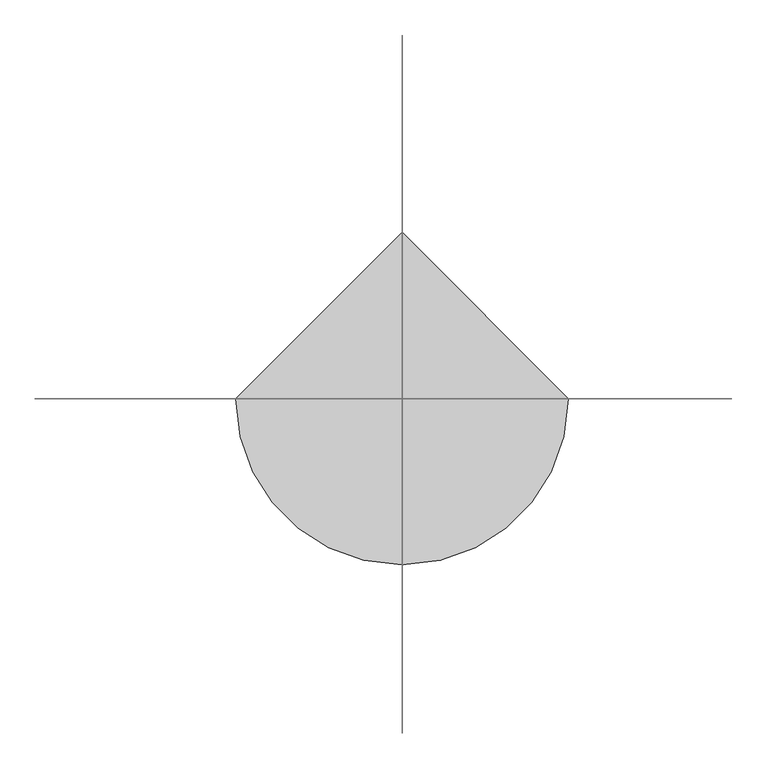
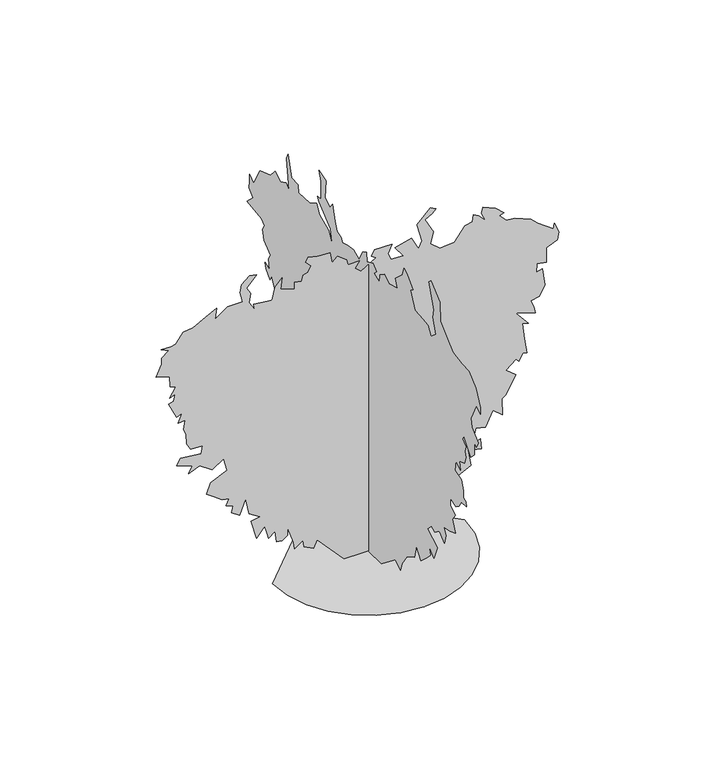
"""IFC4 building model written with IfcOpenShell, lengths in millimetres: proxy geometry, meadowlark 26084 : meadowlark 26084."""

import ifcopenshell
import ifcopenshell.guid

model = None  # the IFC model being written
_history = None  # IfcOwnerHistory: only IFC2X3 demands one
_inside = {}  # id of a spatial element -> (the spatial element, [elements in it])
_under = {}  # id of a project, library or spatial element -> (it, [spatial elements below it])
_declared = {}  # id of a project -> (the project, [libraries it declares])
_typed = {}  # id of a type object -> (the type object, [elements of that type])
_made_of = {}  # id of a material, layer set ... -> (it, [elements and type objects made of it])


def new_model(schema):
    """Start an empty IFC model of exactly this schema.

    Asked for "IFC4X3", IfcOpenShell would pick the latest addendum, in which some entities
    have other attributes; the version numbers below select the first issue.
    IFC2X3 requires an IfcOwnerHistory on every rooted entity: one is made here for all.
    """
    global model, _history
    if schema == "IFC4X3":
        model = ifcopenshell.file(schema_version=(4, 3, 0, 0))
    else:
        model = ifcopenshell.file(schema=schema)
    _inside.clear()
    _under.clear()
    _declared.clear()
    _typed.clear()
    _made_of.clear()
    _history = None
    if model.schema == "IFC2X3":
        org = make("IfcOrganization", Name="unknown")
        user = make(
            "IfcPersonAndOrganization",
            ThePerson=make("IfcPerson", FamilyName="unknown"),
            TheOrganization=org,
        )
        app = make(
            "IfcApplication",
            ApplicationDeveloper=org,
            Version="unknown",
            ApplicationFullName="unknown",
            ApplicationIdentifier="unknown",
        )
        _history = make(
            "IfcOwnerHistory",
            OwningUser=user,
            OwningApplication=app,
            ChangeAction="ADDED",
            CreationDate=0,
        )
    return model


def make(cls, **values):
    """One entity of the class cls with the attributes given. An attribute that is None is left unset."""
    return model.create_entity(
        cls, **{name: value for name, value in values.items() if value is not None}
    )


def rooted(cls, **values):
    """An entity with a GlobalId (a new one), such as an element, a storey or a relation."""
    return make(cls, GlobalId=ifcopenshell.guid.new(), OwnerHistory=_history, **values)


def si_unit(unit_type, name, prefix=None):
    """IfcSIUnit, for example si_unit("LENGTHUNIT", "METRE", prefix="MILLI")."""
    return make("IfcSIUnit", UnitType=unit_type, Prefix=prefix, Name=name)


def assignment(units):
    """IfcUnitAssignment: the units of a project."""
    return None if units is None else make("IfcUnitAssignment", Units=units)


def point(xyz):
    """IfcCartesianPoint."""
    return None if xyz is None else make("IfcCartesianPoint", Coordinates=xyz)


def direction(xyz):
    """IfcDirection."""
    return None if xyz is None else make("IfcDirection", DirectionRatios=xyz)


def frame(location, z_axis=None, x_axis=None):
    """IfcAxis2Placement3D, a coordinate frame: its origin and axes. An axis left out is left unset."""
    return make(
        "IfcAxis2Placement3D",
        Location=point(location),
        Axis=direction(z_axis),
        RefDirection=direction(x_axis),
    )


def origin():
    """The frame at (0, 0, 0) with its axes left unset."""
    return frame((0.0, 0.0, 0.0))


def place(relative_to, where):
    """IfcLocalPlacement: puts the frame where relative to a parent placement (None: the world)."""
    return make(
        "IfcLocalPlacement", PlacementRelTo=relative_to, RelativePlacement=where
    )


def context(
    kind, dimensions, precision=None, world=None, true_north=None, identifier=None
):
    """IfcGeometricRepresentationContext, for example the 3D "Model" context."""
    return make(
        "IfcGeometricRepresentationContext",
        ContextIdentifier=identifier,
        ContextType=kind,
        CoordinateSpaceDimension=dimensions,
        Precision=precision,
        WorldCoordinateSystem=world,
        TrueNorth=true_north,
    )


def project(units=None, contexts=None):
    """IfcProject with its units and contexts."""
    return rooted(
        "IfcProject",
        Name="project",
        RepresentationContexts=contexts,
        UnitsInContext=assignment(units),
    )


def spatial(cls, under=None, at=None, **own):
    """A site, building, storey or space (cls), placed at a placement, below another one or the project."""
    s = rooted(cls, ObjectPlacement=at, **own)
    if under is not None:
        _under.setdefault(under.id(), (under, []))[1].append(s)
    return s


def point_list(points):
    """IfcCartesianPointList2D or 3D."""
    cls = (
        "IfcCartesianPointList2D" if len(points[0]) == 2 else "IfcCartesianPointList3D"
    )
    return make(cls, CoordList=points)


def triangles(points, corners, closed=None, point_numbers=None):
    """IfcTriangulatedFaceSet: each triangle names its three corners, points numbered from 1."""
    return make(
        "IfcTriangulatedFaceSet",
        Coordinates=point_list(points),
        Closed=closed,
        CoordIndex=corners,
        PnIndex=point_numbers,
    )


def shape(context_of_items, identifier, shape_type, items):
    """IfcShapeRepresentation: the items that make up one representation, for example the "Body"."""
    return make(
        "IfcShapeRepresentation",
        ContextOfItems=context_of_items,
        RepresentationIdentifier=identifier,
        RepresentationType=shape_type,
        Items=items,
    )


def source(mapping_origin, context_of_items, identifier, shape_type, items):
    """IfcRepresentationMap: a shape defined once, which mapped items show again and again."""
    return make(
        "IfcRepresentationMap",
        MappingOrigin=mapping_origin,
        MappedRepresentation=shape(context_of_items, identifier, shape_type, items),
    )


def transform(
    local_origin,
    x_axis=None,
    y_axis=None,
    z_axis=None,
    scale=None,
    scale2=None,
    scale3=None,
    uniform=True,
):
    """IfcCartesianTransformationOperator3D, or its non-uniform kind. x_axis, y_axis, z_axis: its Axis1, 2, 3."""
    if uniform:
        return make(
            "IfcCartesianTransformationOperator3D",
            Axis1=direction(x_axis),
            Axis2=direction(y_axis),
            LocalOrigin=point(local_origin),
            Scale=scale,
            Axis3=direction(z_axis),
        )
    return make(
        "IfcCartesianTransformationOperator3DnonUniform",
        Axis1=direction(x_axis),
        Axis2=direction(y_axis),
        LocalOrigin=point(local_origin),
        Scale=scale,
        Axis3=direction(z_axis),
        Scale2=scale2,
        Scale3=scale3,
    )


def mapped(mapping_source, mapping_target):
    """IfcMappedItem: shows the shape of a source again, moved by a transform."""
    return make(
        "IfcMappedItem", MappingSource=mapping_source, MappingTarget=mapping_target
    )


def made_of(thing, what):
    """Note that an element or type object is made of a material, layer set ...; save() writes the relation."""
    if what is not None:
        _made_of.setdefault(what.id(), (what, []))[1].append(thing)
    return thing


def element(
    cls,
    number,
    at=None,
    inside=None,
    cuts=None,
    type_object=None,
    material=None,
    context=None,
    identifier="Body",
    shape_type=None,
    held_by="IfcProductDefinitionShape",
    body=None,
    shapes=None,
    **own,
):
    """One element of the class cls, such as IfcWall. Its Tag is "e" and its number.

    at: its placement. inside: the storey or other place that contains it. cuts: it is an
    opening in that element (IfcRelVoidsElement). A single representation is given by context,
    identifier, shape_type and body (its items); several are given by shapes. held_by: the class
    of the entity that holds the representations. save() writes the other relations.
    """
    e = rooted(cls, Tag="e%d" % number, ObjectPlacement=at, **own)
    if body is not None:
        shapes = [shape(context, identifier, shape_type, body)]
    if shapes is not None:
        e.Representation = make(held_by, Representations=shapes)
    if inside is not None:
        _inside.setdefault(inside.id(), (inside, []))[1].append(e)
    if cuts is not None:
        rooted(
            "IfcRelVoidsElement", RelatingBuildingElement=cuts, RelatedOpeningElement=e
        )
    if type_object is not None:
        _typed.setdefault(type_object.id(), (type_object, []))[1].append(e)
    return made_of(e, material)


def aggregate(whole, parts):
    """IfcRelAggregates: a whole, such as a stair, and the parts it consists of."""
    return rooted("IfcRelAggregates", RelatingObject=whole, RelatedObjects=parts)


def save(model, path):
    """Write the relations noted so far, then the file.

    IfcRelAggregates (storeys below a building ...), IfcRelContainedInSpatialStructure (elements
    in a storey), IfcRelDefinesByType, IfcRelAssociatesMaterial and IfcRelDeclares: one each for
    every whole, place, type object, material and project.
    """
    for whole, parts in _under.values():
        aggregate(whole, parts)
    for where, things in _inside.values():
        rooted(
            "IfcRelContainedInSpatialStructure",
            RelatedElements=things,
            RelatingStructure=where,
        )
    for kind, things in _typed.values():
        rooted("IfcRelDefinesByType", RelatedObjects=things, RelatingType=kind)
    for what, things in _made_of.values():
        rooted("IfcRelAssociatesMaterial", RelatedObjects=things, RelatingMaterial=what)
    for by, libraries in _declared.values():
        rooted("IfcRelDeclares", RelatingContext=by, RelatedDefinitions=libraries)
    model.write(path)


def entourage_9ef344a8(model_context):
    return source(origin(), model_context, "Body", "Tessellation", [
        triangles([(-63.9369313, 2.6e-06, 2.5813025), (-98.6351404, 1.9e-06, 41.3616468), (-133.3335948, 1.1e-06, 80.1421467), (-143.538813, 2.7e-06, 59.7314513), (-168.0315495, 3.1e-06, 71.9778149), (-170.0726858, 2.1e-06, 90.347365), (-192.5245312, 3.9e-06, 76.0598514), (-194.5656857, 2.9e-06, 94.4296558), (-210.8940858, 9e-07, 139.3333375), (-210.8940858, 2.1e-06, 118.9223832), (-225.1818402, 3.4e-06, 108.7171649), (-239.469104, 3.9e-06, 110.7583103), (-243.5513948, 2.2e-06, 141.3742286), (-260.2917792, 3.7e-06, 128.4682213), (-264.2033864, 3e-06, 143.1357217), (-270.0860397, 2e-06, 163.8260649), (-290.4949502, 4.4e-06, 139.3333375), (-304.7824684, 2e-06, 190.3599468), (-282.331386, 8e-07, 194.4422376), (-310.9064223, 9e-07, 212.8117922), (-319.0699865, -1.4e-06, 257.7162279), (-335.3996584, 1.7e-06, 216.894083), (-355.8110942, 1.8e-06, 231.181583), (-351.7293303, 5e-07, 249.5511376), (-370.0986305, 9e-07, 255.674056), (-361.9325229, -4e-07, 272.003746), (-380.3043303, 2e-07, 276.0855281), (-401.9400736, 2e-07, 291.703997), (-421.1247311, 3e-07, 304.6605463), (-410.918995, -1.9e-06, 333.2355826), (-368.1987102, -4.9e-06, 351.9401459), (-376.2200229, -6.6e-06, 386.3038187), (-406.8371947, -4.1e-06, 367.9345184), (-439.493995, -4.1e-06, 390.385619), (-468.0690313, -2.1e-06, 378.137711), (-457.8632953, -3.5e-06, 394.4673829), (-498.6862032, -2.7e-06, 410.7970548), (-488.4805035, -4.1e-06, 427.1242195), (-435.4122311, -6.1e-06, 421.0002474), (-431.3304308, -7.5e-06, 441.4117195), (-461.9450955, -6.2e-06, 443.4538914), (-472.1508316, -6.9e-06, 461.8231553), (-474.1929671, -8.4e-06, 488.3560198), (-480.3169393, -9e-06, 502.6435561), (-476.2325955, -1.06e-05, 527.1367922), (-495.4832737, -9.7e-06, 526.35192), (-484.3987032, -1.16e-05, 549.5878564), (-498.6862032, -1.06e-05, 543.466464), (-519.0951319, -1.23e-05, 586.3290004), (-506.8497674, -1.3e-05, 590.4107643), (-502.7680035, -1.43e-05, 608.7800646), (-517.0555035, -1.33e-05, 602.6561288), (-500.7258316, -1.55e-05, 627.1493649), (-516.1995237, -1.52e-05, 634.2689884), (-517.0555035, -1.68e-05, 661.848337), (-551.7544756, -1.59e-05, 672.0540367), (-537.4644321, -1.84e-05, 702.6687378), (-538.1857907, -1.94e-05, 720.3319038), (-519.0951319, -2.1e-05, 733.2859097), (-539.506604, -2.07e-05, 743.4916094), (-512.7375257, -2.18e-05, 742.0895147), (-500.7258316, -2.25e-05, 745.5312378), (-482.3565313, -2.49e-05, 772.0666094), (-455.8236669, -2.62e-05, 774.1062378), (-423.1668666, -2.87e-05, 792.4755381), (-395.1176339, -3.08e-05, 806.3871162), (-398.6736305, -2.9e-05, 778.1880381), (-366.0168303, -3.17e-05, 800.6416821), (-327.2360942, -3.34e-05, 800.6416821), (-334.4166515, -3.47e-05, 827.9339842), (-330.1088113, -3.62e-05, 849.0616917), (-308.8667939, -3.81e-05, 865.9552826), (-290.4949502, -3.87e-05, 861.8734823), (-317.5358142, -3.58e-05, 834.0731443), (-306.8246221, -3.53e-05, 816.9688105), (-310.9064223, -3.36e-05, 792.4755381), (-296.6189042, -3.29e-05, 770.0245102), (-298.6610579, -3.37e-05, 784.3120102), (-251.0357672, -3.54e-05, 778.383593), (-243.5513948, -3.77e-05, 810.8473818), (-225.1818402, -3.97e-05, 831.2563105), (-228.2958943, -3.78e-05, 801.312208), (-192.5245312, -3.86e-05, 788.3937378), (-192.5245312, -3.97e-05, 806.7630381), (-173.5245645, -4.03e-05, 803.1613684), (-170.0726858, -4.14e-05, 819.0109823), (-157.8260678, -4.22e-05, 823.0927099), (-149.662004, -4.34e-05, 837.3802826), (-163.9495131, -4.36e-05, 851.6677826), (-157.8260678, -4.46e-05, 863.9131107), (-131.292195, -4.54e-05, 857.7916821), (-100.6760314, -4.66e-05, 855.7495102), (-94.5528496, -4.52e-05, 827.1745102), (-80.2653314, -4.65e-05, 839.4223818), (-56.9158573, -4.65e-05, 821.1673914), (-53.7314587, -4.57e-05, 806.7630381), (-23.1153655, -4.71e-05, 806.7630381), (-35.3616542, -4.56e-05, 790.4359097), (-19.0331746, -4.54e-05, 776.1484097), (19.7470164, -4.86e-05, 800.6416821), (7.5007532, -4.85e-05, 808.8052099), (15.1231208, -4.98e-05, 823.890263), (60.5683824, -5.17e-05, 823.0927099), (50.5958261, -4.99e-05, 799.816151), (58.5274868, -4.92e-05, 782.2723818), (91.1845505, -5.05e-05, 780.2302099), (68.732964, -5.13e-05, 810.8473818), (111.5952414, -5.38e-05, 821.0506107), (129.9650504, -5.25e-05, 786.3541821), (138.9452253, -5.4e-05, 804.6625122), (125.8830048, -5.64e-05, 853.7099545), (160.581223, -6e-05, 888.4063831), (174.868723, -6.01e-05, 880.2427826), (164.6635138, -5.91e-05, 870.0370829), (146.2937048, -5.76e-05, 859.8313105), (168.7455503, -5.62e-05, 819.0109823), (161.0930195, -5.4e-05, 788.6985884), (185.0742047, -5.39e-05, 767.9848818), (203.4434868, -5.48e-05, 770.0245102), (223.8544503, -5.58e-05, 772.0666094), (250.3885683, -5.9e-05, 806.7630381), (269.7101179, -6.01e-05, 811.2766434), (272.8393963, -6.13e-05, 829.2166821), (285.0872861, -6.15e-05, 823.0927099), (304.0839645, -6.12e-05, 803.1613684), (293.2508503, -6.21e-05, 827.1745102), (297.3326324, -6.31e-05, 841.4620102), (329.9894508, -6.37e-05, 827.1745102), (351.394031, -6.35e-05, 807.9441433), (340.0529354, -6.27e-05, 803.4457987), (358.5644508, -6.24e-05, 784.3120102), (381.0180948, -6.33e-05, 782.2723818), (422.1051581, -6.41e-05, 765.7470823), (440.2077596, -6.38e-05, 747.5734097), (481.0306675, -6.39e-05, 718.9984097), (483.0702959, -6.48e-05, 733.2859097), (495.3181675, -6.36e-05, 704.710837), (491.2364036, -6.23e-05, 684.2994375), (462.6588238, -6.03e-05, 672.0540367), (462.6588238, -5.8e-05, 633.273337), (438.1681312, -5.71e-05, 637.3550646), (436.1259593, -5.57e-05, 614.9040367), (452.4556312, -5.67e-05, 618.9857643), (458.5770598, -5.41e-05, 572.041464), (444.2895235, -5.19e-05, 545.5060925), (421.8384593, -5.07e-05, 541.4242922), (430.0020235, -4.98e-05, 521.0128201), (434.0863309, -4.91e-05, 504.6856916), (383.0577232, -4.78e-05, 521.0128201), (415.7145235, -4.69e-05, 482.2346274), (399.3873951, -4.64e-05, 486.3163914), (405.5087874, -4.42e-05, 443.4538914), (411.6327232, -4.2e-05, 402.6309471), (401.4269872, -4.17e-05, 404.673119), (391.2212874, -4.01e-05, 386.3038187), (383.0577232, -4.03e-05, 394.4673829), (356.5248588, -3.79e-05, 374.0559471), (383.0577232, -3.77e-05, 351.6048466), (356.5248588, -3.39e-05, 306.7001747), (346.3191227, -3.29e-05, 298.5365923), (348.3587511, -3.03e-05, 253.6334284), (323.4463909, -3.05e-05, 274.9933165), (303.4565864, -2.73e-05, 235.2636194), (278.9633503, -2.66e-05, 241.3868104), (266.8272088, -2.35e-05, 199.2829668), (291.2086966, -2.52e-05, 208.7297557), (293.2508503, -2.36e-05, 180.1547194), (258.5518782, -2.25e-05, 188.3190466), (266.7179858, -2.02e-05, 143.415374), (232.0187775, -1.77e-05, 127.0867195), (215.6903774, -1.54e-05, 100.5528377), (197.3205684, -1.5e-05, 106.6760195), (191.1973775, -1.2e-05, 61.7723423), (176.9098775, -1.3e-05, 88.306474), (150.3759956, -8.8e-06, 37.2796104), (132.0059414, -8.8e-06, 51.5671195), (68.732964, -3.2e-06, 2.5813025), (5e-07, 58.5086925, 0.0), (5.6e-06, 119.7410287, 55.1089), (6.1e-06, 137.5863239, 49.658565), (5.6e-06, 170.7679014, 104.0948725), (5.5e-06, 180.9731106, 91.8482545), (9.8e-06, 197.3017651, 73.4787044), (6.8e-06, 213.6304195, 87.7662181), (6.7e-06, 205.4660923, 93.8893999), (9.7e-06, 223.8356469, 144.9162635), (8.6e-06, 231.9999742, 112.2589454), (1e-05, 238.1231651, 136.7519272), (1.13e-05, 276.9033925, 128.5875999), (1.12e-05, 254.4523283, 148.9982999), (1.22e-05, 274.8637822, 151.0394453), (1.45e-05, 307.5205825, 171.4501453), (1.42e-05, 280.9851927, 191.8608363), (1.68e-05, 299.3544748, 232.6824725), (1.68e-05, 317.7263186, 214.3126635), (1.89e-05, 350.3043809, 228.0708535), (1.99e-05, 340.1773828, 261.2569819), (2.07e-05, 354.4649191, 265.338764), (2.22e-05, 356.5045112, 297.9955825), (2.36e-05, 393.2456552, 293.9138004), (2.61e-05, 411.6149554, 332.6945546), (2.58e-05, 397.3274554, 338.8184904), (2.92e-05, 438.1478199, 377.5992265), (2.82e-05, 405.4910196, 385.7627907), (2.9e-05, 411.6149554, 398.0081552), (2.55e-05, 417.7363478, 412.2956552), (2.48e-05, 395.2852836, 418.4196273), (2.73e-05, 415.6967194, 455.1581915), (2.98e-05, 436.1081915, 491.8993355), (2.95e-05, 444.2717557, 477.6118355), (3.11e-05, 460.5988841, 498.0207278), (3.2e-05, 466.7228199, 512.3082642), (3.07e-05, 446.3113841, 504.1447), (3.21e-05, 450.3956915, 530.6800715), (3.24e-05, 440.1899554, 547.0072), (3.47e-05, 470.8046202, 569.4583005), (3.61e-05, 476.928556, 595.9937084), (3.64e-05, 468.7649918, 610.2812084), (3.74e-05, 481.0103562, 622.5265366), (4.07e-05, 546.3265002, 630.6926805), (4.07e-05, 519.7910923, 657.2255087), (4.22e-05, 538.1603926, 673.5551805), (4.29e-05, 536.5677936, 692.1911797), (4.37e-05, 535.3943187, 712.0133709), (4.23e-05, 517.7489204, 698.0459095), (3.89e-05, 487.134292, 751.1141819), (3.76e-05, 440.1899554, 767.4438538), (3.77e-05, 419.7785196, 789.8948816), (3.6e-05, 395.2852836, 775.6073816), (3.55e-05, 370.7920475, 787.8553259), (3.44e-05, 358.546683, 775.6073816), (3.84e-05, 368.7524191, 857.250654), (3.88e-05, 362.6284833, 871.5382267), (3.56e-05, 346.2988114, 816.4303259), (3.43e-05, 317.7237751, 814.388154), (3.33e-05, 315.6841467, 793.9766819), (3.12e-05, 262.6158925, 798.0584822), (3.06e-05, 234.0411286, 814.388154), (2.9e-05, 219.7536105, 791.9370535), (2.65e-05, 180.9731106, 773.5677532), (2.43e-05, 162.603556, 740.9084095), (2.65e-05, 170.7679014, 783.7709822), (3.06e-05, 223.8356469, 824.5938538), (3.15e-05, 229.9590922, 836.8392546), (3.08e-05, 213.6301652, 838.8814264), (3.3e-05, 213.6301652, 887.8678986), (3.45e-05, 223.8356469, 912.3585548), (3.26e-05, 191.1785923, 902.1553986), (3.06e-05, 195.2606287, 853.1689264), (2.91e-05, 172.8087833, 840.9209822), (2.93e-05, 162.603556, 855.2085548), (2.71e-05, 150.356947, 816.4303259), (2.57e-05, 142.1926198, 793.9766819), (2.47e-05, 123.8230652, 787.8553259), (2.4e-05, 117.7001377, 777.6495535), (2.32e-05, 95.248047, 783.7709822), (2.23e-05, 68.7141651, 787.8553259), (2.06e-05, 43.1368564, 776.3617687), (2.13e-05, 25.8518877, 808.2641819), (2.09e-05, 9.5229755, 816.4303259), (1.98e-05, 7.4819061, 791.9370535), (1.91e-05, -19.0520211, 804.1824543), (1.78e-05, -35.3804508, 789.8948816), (1.78e-05, -25.1750781, 779.6891819), (1.63e-05, -49.6682165, 769.4834822), (1.72e-05, -51.7091075, 791.9370535), (1.69e-05, -72.1200574, 806.2245535), (1.54e-05, -92.5307528, 791.9370535), (1.42e-05, -129.2700982, 802.1428259), (1.56e-05, -121.105771, 824.5938538), (1.54e-05, -153.0015985, 852.691412), (1.61e-05, -159.8860075, 875.6199543), (1.52e-05, -172.1326437, 867.4564264), (1.28e-05, -200.7076618, 840.9209822), (1.3e-05, -188.4607894, 832.7574543), (1.02e-05, -208.8717347, 789.8948816), (8.5e-06, -245.6110801, 787.8553259), (7.4e-06, -268.0641973, 783.7709822), (5.8e-06, -280.3095436, 761.3198816), (5.7e-06, -303.1314609, 780.7331589), (8e-06, -290.5152796, 820.5121262), (8.8e-06, -294.5970617, 842.963154), (1.25e-05, -272.1459794, 906.2371988), (1.25e-05, -280.3095436, 914.4007267), (9.2e-06, -321.1299262, 879.7017546), (6.9e-06, -323.1720617, 828.675654), (4.3e-06, -354.6452497, 799.5291046), (2.2e-06, -380.3221344, 777.6495535), (1e-07, -421.1424989, 771.5255814), (-1.3e-06, -451.7596707, 769.4834822), (-3.9e-06, -482.3768789, 740.9084095), (-6.6e-06, -502.7857713, 700.0880814), (-7.4e-06, -502.7857713, 681.7187811), (-6e-06, -486.4586429, 696.0062811), (-2.7e-06, -459.9232349, 644.9801805), (-3.9e-06, -466.0472071, 624.5687084), (-6.3e-06, -494.6222071, 598.0333005), (-6.6e-06, -486.4586429, 581.7061721), (-5.9e-06, -476.2529068, 587.8301442), (-7.3e-06, -476.2529068, 555.1708005), (-7.3e-06, -459.9232349, 538.8436357), (-4.3e-06, -429.3086065, 577.6244081), (-4.5e-06, -423.1846707, 567.4186721), (-5.7e-06, -439.5143426, 555.1708005), (-6.2e-06, -433.3903705, 538.8436357), (-7.1e-06, -439.5143426, 524.5561357), (-7.6e-06, -431.3482349, 504.1447), (-7e-06, -408.8971344, 495.9810994), (-8.2e-06, -412.9789347, 473.5300352), (-6.6e-06, -392.5674625, 487.8175352), (-7.7e-06, -388.4856986, 459.2425352), (-9.4e-06, -419.1028705, 451.0764276), (-1.08e-05, -427.2664347, 426.5831915), (-1.17e-05, -428.2418112, 408.450105), (-1.23e-05, -437.4721707, 402.0924989), (-1.3e-05, -441.553971, 391.8867628), (-1.21e-05, -419.1028705, 389.844591), (-1.23e-05, -406.8549989, 371.4752907), (-1.22e-05, -394.6096344, 363.3117265), (-1.07e-05, -368.0767699, 369.4331188), (-7.3e-06, -368.0767699, 349.0242265), (-8.8e-06, -390.5278705, 336.7763186), (-9e-06, -378.2799625, 318.4070183), (-1.09e-05, -390.5278705, 287.7923899), (-1.03e-05, -366.0345981, 277.5866538), (-9.3e-06, -339.5017336, 273.5048717), (-1.05e-05, -347.6653341, 255.1330462), (-1.13e-05, -341.541362, 230.6413362), (-9.5e-06, -319.0902978, 249.0108726), (-9.2e-06, -298.6788438, 234.7233726), (-8.2e-06, -284.3913257, 242.8876998), (-8.2e-06, -266.0220254, 224.5181452), (-1.13e-05, -310.9241901, 200.0251635), (-1.22e-05, -294.5970617, 161.2446636), (-1.04e-05, -272.1459794, 181.6556089), (-1.16e-05, -278.2673899, 159.2037635), (-1.17e-05, -263.9798717, 142.8751181), (-1.15e-05, -235.4058709, 118.3821273), (-9.5e-06, -214.9951618, 144.9162635), (-1.06e-05, -205.8577653, 109.83274), (-1e-05, -174.1735256, 91.8482545), (-1.05e-05, -149.6807982, 57.1500454), (-6.7e-06, -143.5573621, 36.7393522), (-5.1e-06, -121.105771, 51.0268636), (-4.5e-06, -57.8322894, 2.0410923), (-249.8274834, 0.0, 0.0911396), (-243.2227266, -57.2440259, 0.0911358), (-224.4129918, -109.8131736, 0.091132), (-194.9037465, -156.2020027, 0.0911279), (-156.2020027, -194.9037465, 0.0911238), (-109.8131736, -224.4127374, 0.09112), (-57.2437715, -243.2227266, 0.0911167), (8.9e-06, -249.8274834, 0.0911137), (57.2440259, -243.2227266, 0.0911116), (109.8131736, -224.4127374, 0.0911454), (156.2020027, -194.9037465, 0.0911452), (194.9040008, -156.2020027, 0.0911459), (224.4127374, -109.8131736, 0.0911122), (243.2227266, -57.2437715, 0.0911147), (249.8274834, 2.18e-05, 0.0911177), (-3.49e-05, 249.8274834, 0.0911434)], [[59, 60, 61], [135, 136, 137], [51, 52, 53], [34, 35, 36], [149, 150, 151], [80, 81, 82], [172, 173, 174], [160, 161, 162], [96, 97, 98], [16, 17, 18], [16, 18, 19], [65, 66, 67], [147, 148, 149], [72, 73, 74], [71, 72, 74], [70, 71, 74], [45, 46, 47], [128, 129, 130], [6, 7, 8], [106, 107, 108], [106, 108, 109], [13, 14, 15], [102, 103, 104], [146, 147, 149], [152, 153, 154], [79, 80, 82], [166, 167, 168], [165, 166, 168], [122, 123, 124], [154, 155, 156], [112, 113, 114], [111, 112, 114], [111, 114, 115], [77, 78, 79], [21, 22, 23], [21, 23, 24], [83, 84, 85], [174, 175, 176], [36, 37, 38], [36, 38, 39], [34, 36, 39], [139, 140, 141], [55, 56, 57], [24, 25, 26], [126, 127, 128], [125, 126, 128], [125, 128, 130], [101, 102, 104], [100, 101, 104], [48, 49, 50], [47, 48, 50], [142, 143, 144], [3, 4, 5], [3, 5, 6], [110, 111, 115], [110, 115, 116], [110, 116, 117], [109, 110, 117], [69, 70, 74], [69, 74, 75], [69, 75, 76], [122, 124, 125], [157, 158, 159], [21, 24, 26], [93, 94, 95], [162, 163, 164], [170, 171, 172], [89, 90, 91], [88, 89, 91], [28, 29, 30], [28, 30, 31], [27, 28, 31], [26, 27, 31], [168, 169, 170], [11, 12, 13], [10, 11, 13], [9, 10, 13], [91, 92, 93], [88, 91, 93], [87, 88, 93], [13, 15, 16], [93, 95, 96], [21, 26, 31], [32, 33, 34], [32, 34, 39], [32, 39, 40], [79, 82, 83], [100, 104, 105], [53, 54, 55], [6, 8, 9], [64, 65, 67], [85, 86, 87], [57, 58, 59], [99, 100, 105], [55, 57, 59], [40, 41, 42], [40, 42, 43], [135, 137, 138], [135, 138, 139], [134, 135, 139], [142, 144, 145], [142, 145, 146], [152, 154, 156], [134, 139, 141], [157, 159, 160], [142, 146, 149], [62, 63, 64], [177, 1, 2], [176, 177, 2], [176, 2, 3], [85, 87, 93], [19, 20, 21], [125, 130, 131], [133, 134, 141], [132, 133, 141], [131, 132, 141], [174, 176, 3], [109, 117, 118], [85, 93, 96], [85, 96, 98], [83, 85, 98], [125, 131, 141], [125, 141, 142], [125, 142, 149], [122, 125, 149], [121, 122, 149], [120, 121, 149], [119, 120, 149], [118, 119, 149], [83, 98, 99], [47, 50, 51], [172, 174, 3], [59, 61, 62], [55, 59, 62], [55, 62, 64], [55, 64, 67], [53, 55, 67], [9, 13, 16], [9, 16, 19], [157, 160, 162], [168, 170, 172], [168, 172, 3], [165, 168, 3], [164, 165, 3], [164, 3, 6], [164, 6, 9], [164, 9, 19], [164, 19, 21], [164, 21, 31], [164, 31, 32], [162, 164, 32], [157, 162, 32], [157, 32, 40], [157, 40, 43], [157, 43, 44], [157, 44, 45], [157, 45, 47], [157, 47, 51], [157, 51, 53], [157, 53, 67], [157, 67, 68], [156, 157, 68], [152, 156, 68], [109, 118, 149], [106, 109, 149], [105, 106, 149], [99, 105, 149], [99, 149, 151], [99, 151, 152], [83, 99, 152], [79, 83, 152], [77, 79, 152], [77, 152, 68], [77, 68, 69], [76, 77, 69], [186, 187, 188], [188, 189, 190], [232, 233, 234], [231, 232, 234], [308, 309, 310], [211, 212, 213], [292, 293, 294], [246, 247, 248], [219, 220, 221], [246, 248, 249], [245, 246, 249], [250, 251, 252], [223, 224, 225], [202, 203, 204], [327, 328, 329], [259, 260, 261], [209, 210, 211], [209, 211, 213], [191, 192, 193], [243, 244, 245], [333, 334, 335], [332, 333, 335], [271, 272, 273], [315, 316, 317], [314, 315, 317], [342, 343, 344], [273, 274, 275], [258, 259, 261], [291, 292, 294], [271, 273, 275], [183, 184, 185], [182, 183, 185], [326, 327, 329], [205, 206, 207], [300, 301, 302], [299, 300, 302], [321, 322, 323], [297, 298, 299], [296, 297, 299], [262, 263, 264], [261, 262, 264], [296, 299, 302], [337, 338, 339], [200, 201, 202], [199, 200, 202], [323, 324, 325], [242, 243, 245], [242, 245, 249], [242, 249, 250], [242, 250, 252], [242, 252, 253], [237, 238, 239], [283, 284, 285], [282, 283, 285], [282, 285, 286], [281, 282, 286], [280, 281, 286], [280, 286, 287], [195, 196, 197], [194, 195, 197], [241, 242, 253], [241, 253, 254], [241, 254, 255], [234, 235, 236], [231, 234, 236], [227, 228, 229], [190, 191, 193], [179, 180, 181], [303, 304, 305], [229, 230, 231], [270, 271, 275], [269, 270, 275], [269, 275, 276], [197, 198, 199], [266, 267, 268], [265, 266, 268], [222, 223, 225], [221, 222, 225], [186, 188, 190], [182, 185, 186], [181, 182, 186], [204, 205, 207], [329, 330, 331], [323, 325, 326], [280, 287, 288], [321, 323, 326], [311, 312, 313], [335, 336, 337], [335, 337, 339], [332, 335, 339], [295, 296, 302], [277, 278, 279], [219, 221, 225], [219, 225, 226], [219, 226, 227], [219, 227, 229], [218, 219, 229], [218, 229, 231], [186, 190, 193], [306, 307, 308], [305, 306, 308], [303, 305, 308], [303, 308, 310], [311, 313, 314], [311, 314, 317], [311, 317, 318], [311, 318, 319], [311, 319, 320], [339, 340, 341], [258, 261, 264], [345, 178, 179], [344, 345, 179], [344, 179, 181], [216, 217, 218], [215, 216, 218], [215, 218, 231], [215, 231, 236], [215, 236, 237], [215, 237, 239], [215, 239, 240], [215, 240, 241], [341, 342, 344], [341, 344, 181], [339, 341, 181], [332, 339, 181], [332, 181, 186], [332, 186, 193], [332, 193, 194], [331, 332, 194], [279, 280, 288], [290, 291, 294], [289, 290, 294], [289, 294, 295], [288, 289, 295], [279, 288, 295], [279, 295, 302], [279, 302, 303], [279, 303, 310], [213, 214, 215], [209, 213, 215], [209, 215, 241], [208, 209, 241], [207, 208, 241], [326, 329, 331], [321, 326, 331], [321, 331, 194], [320, 321, 194], [311, 320, 194], [310, 311, 194], [279, 310, 194], [277, 279, 194], [276, 277, 194], [269, 276, 194], [268, 269, 194], [265, 268, 194], [264, 265, 194], [258, 264, 194], [258, 194, 197], [258, 197, 199], [258, 199, 202], [258, 202, 204], [258, 204, 207], [258, 207, 241], [258, 241, 255], [258, 255, 256], [257, 258, 256], [360, 361, 346], [359, 360, 346], [359, 346, 347], [358, 359, 347], [358, 347, 348], [358, 348, 349], [357, 358, 349], [356, 357, 349], [356, 349, 350], [356, 350, 351], [356, 351, 352], [356, 352, 353], [356, 353, 354], [356, 354, 355]], closed=False),
    ])


if __name__ == "__main__":
    model = new_model("IFC4")
    model_context = context("Model", 3, world=origin())
    ifc_project = project(units=[si_unit("LENGTHUNIT", "METRE", prefix="MILLI")], contexts=[model_context])
    site = spatial("IfcSite", under=ifc_project)
    building = spatial("IfcBuilding", under=site)
    placement = place(None, origin())
    entourage_shape = entourage_9ef344a8(model_context)
    element("IfcBuildingElementProxy", 1, Name="meadowlark 26084 : meadowlark 26084", ObjectType="meadowlark 26084 : meadowlark 26084", at=placement, inside=building, context=model_context, shape_type="MappedRepresentation", body=[
        mapped(entourage_shape, transform((0.0, 0.0, 0.0), x_axis=(1.0, 0.0, 0.0), y_axis=(0.0, 1.0, 0.0), z_axis=(0.0, 0.0, 1.0))),
    ])
    save(model, "model.ifc")

# Revit data of these elements
# Type "meadowlark 26084 : meadowlark 26084"
#   built-in parameter 1005195 = "RPC-16-G0FT-Q7G0-0DUH-W000-ST1L-LVER-AU"
#   Height = 0
